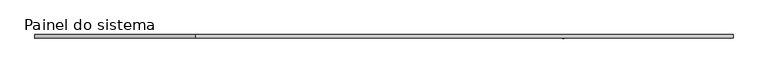
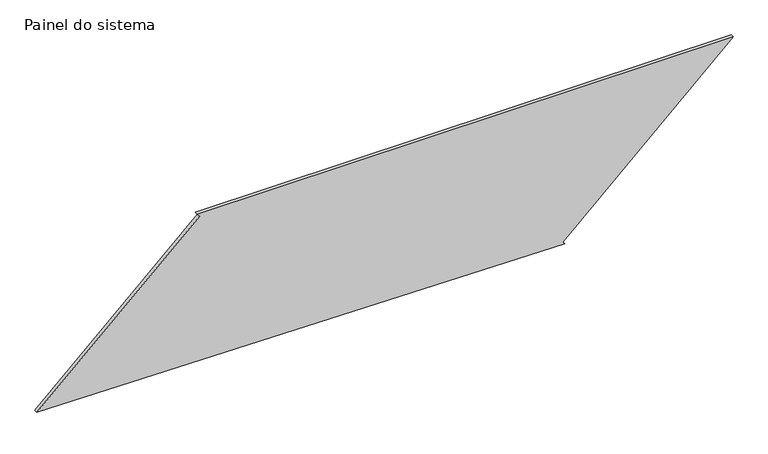
"""IFC4 building model written with IfcOpenShell, lengths in millimetres: plate geometry, Painel do sistema : Envidraçado."""

from ifc_helpers import new_model, si_unit, frame, origin, place, context, project, spatial, polyline, outline, extrude, source, transform, mapped, element, save


def painel_do_sistema_94d4ea3e(model_context):
    return source(origin(), model_context, "Body", "SweptSolid", [
        extrude(outline(polyline([(0.0, 1261.9071137), (18.3764951, 1244.9570569), (1122.0721155, 2441.5345898), (1122.0721155, -1316.0176159), (1103.6956204, -1299.067559), (49.9102838, -2441.5345898), (0.0, 1261.9071137)])), frame((0.0, 24.5, 0.0), z_axis=(0.0, 1.0, 0.0), x_axis=(0.0, 0.0, 1.0)), (0.0, 0.0, 1.0), 25.0),
    ])


if __name__ == "__main__":
    model = new_model("IFC4")
    model_context = context("Model", 3, world=origin())
    ifc_project = project(units=[si_unit("LENGTHUNIT", "METRE", prefix="MILLI")], contexts=[model_context])
    site = spatial("IfcSite", under=ifc_project)
    building = spatial("IfcBuilding", under=site)
    placement = place(None, origin())
    painel_do_sistema_shape = painel_do_sistema_94d4ea3e(model_context)
    element("IfcPlate", 1, ObjectType="Painel do sistema : Envidraçado", at=placement, inside=building, context=model_context, shape_type="MappedRepresentation", body=[
        mapped(painel_do_sistema_shape, transform((0.0, 0.0, 0.0), x_axis=(1.0, 0.0, 0.0), y_axis=(0.0, 1.0, 0.0), z_axis=(0.0, 0.0, 1.0))),
    ])
    save(model, "model.ifc")

# Revit data of these elements
# Type "Painel do sistema : Envidraçado"
#   Construction Type Id = "GSP4R"
#   Analytic Construction = "Vidraça única Pilkington 1/8 pol"
#   Visual Light Transmittance = 0.9
#   Solar Heat Gain Coefficient = 0.86
#   Heat Transfer Coefficient (U) = 6.7069 W/(m²·K)
# Element 1 (IfcPlate, "Painel do sistema : Envidraçado")
#   Materials on its faces: "Vidro"
# Materials
#   "Vidro": class "Vidro", colour RGB 0 128 192, transparency 0.9, Description = "Vidro de sílica", Cost = 0
